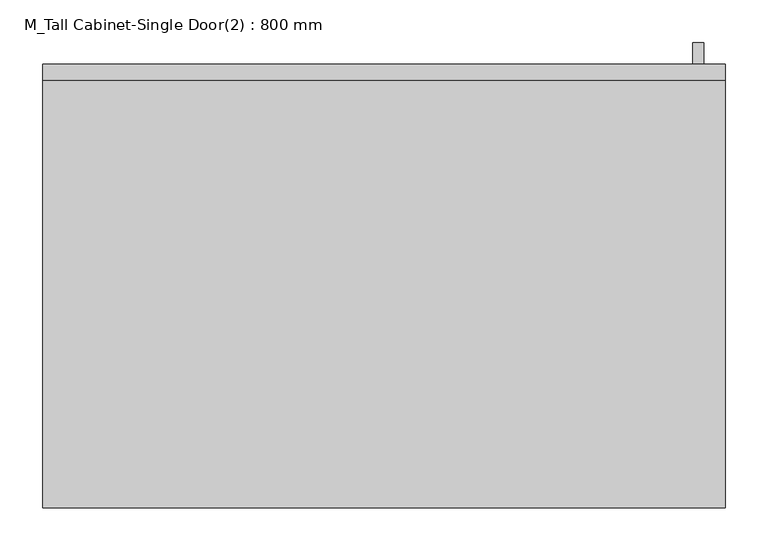
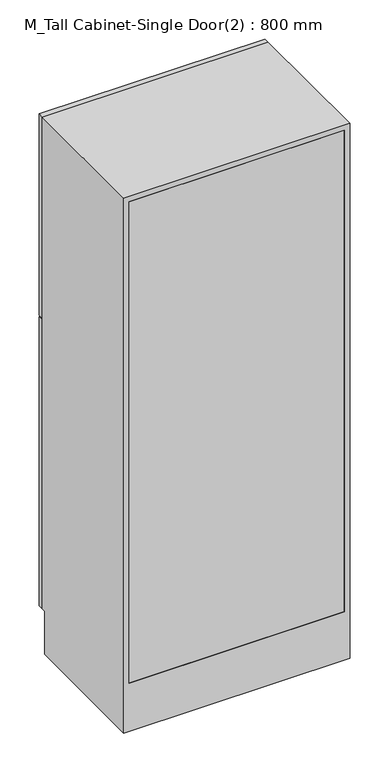
"""IFC4 building model written with IfcOpenShell, lengths in millimetres: furniture geometry, M_Tall Cabinet-Single Door(2) : 800 mm."""

from ifc_helpers import new_model, si_unit, frame, origin, place, context, project, spatial, polyline, outline, extrude, faceted_brep, source, transform, mapped, element, save


def m_tall_cabinet_single_door_2_800_mm_e6cfeb17(model_context):
    return source(origin(), model_context, "Body", "SolidModel", [
        faceted_brep([(418.7377049, 500.95, 161.5875), (-381.2622951, 500.95, 161.5875), (-381.2622951, 500.95, 2000.0), (418.7377049, 500.95, 2000.0), (399.6877049, 500.95, 1980.95), (-362.2122951, 500.95, 1980.95), (-362.2122951, 500.95, 180.6375), (399.6877049, 500.95, 180.6375), (-381.2622951, 0.0, 2000.0), (-381.2622951, 0.0, 0.0), (418.7377049, 0.0, 0.0), (418.7377049, 0.0, 2000.0), (399.6877049, 0.0, 1980.95), (399.6877049, 0.0, 180.6375), (-362.2122951, 0.0, 180.6375), (-362.2122951, 0.0, 1980.95), (418.7377049, 485.0, 0.0), (418.7377049, 485.0, 161.5875), (-381.2622951, 485.0, 161.5875), (-381.2622951, 485.0, 0.0)], [[[0, 1, 2, 3], [4, 5, 6, 7]], [[8, 9, 10, 11], [12, 13, 14, 15]], [[3, 11, 10, 16, 17, 0]], [[2, 8, 11, 3]], [[1, 18, 19, 9, 8, 2]], [[0, 17, 18, 1]], [[7, 13, 12, 4]], [[6, 14, 13, 7]], [[5, 15, 14, 6]], [[4, 12, 15, 5]], [[10, 9, 19, 16]], [[19, 18, 17, 16]]]),
        extrude(outline(polyline([(393.3377049, 545.4), (393.3377049, 520.0), (380.8054733, 520.0), (380.8054733, 545.4), (393.3377049, 545.4)])), frame((0.0, 0.0, 1269.9480367), z_axis=(0.0, 0.0, 1.0), x_axis=(1.0, 0.0, 0.0)), (0.0, 0.0, 1.0), 101.6),
        extrude(outline(polyline([(393.3377049, 545.4), (393.3377049, 520.0), (380.8054733, 520.0), (380.8054733, 545.4), (393.3377049, 545.4)])), frame((0.0, 0.0, 1117.5480367), z_axis=(0.0, 0.0, 1.0), x_axis=(1.0, 0.0, 0.0)), (0.0, 0.0, 1.0), 101.6),
        extrude(outline(polyline([(355.2377049, 507.3), (355.2377049, 500.95), (-317.7622951, 500.95), (-317.7622951, 507.3), (355.2377049, 507.3)])), frame((0.0, 0.0, 1308.0480367), z_axis=(0.0, 0.0, 1.0), x_axis=(1.0, 0.0, 0.0)), (0.0, 0.0, 1.0), 628.4519633),
        extrude(outline(polyline([(355.2377049, 507.3), (355.2377049, 500.95), (-317.7622951, 500.95), (-317.7622951, 507.3), (355.2377049, 507.3)])), frame((0.0, 0.0, 225.0875), z_axis=(0.0, 0.0, 1.0), x_axis=(1.0, 0.0, 0.0)), (0.0, 0.0, 1.0), 955.9605367),
        extrude(outline(polyline([(2000.0, 418.7377049), (2000.0, -381.2622951), (1247.7230367, -381.2622951), (1247.7230367, 418.7377049), (2000.0, 418.7377049)]), holes=[polyline([(1936.5, 355.2377049), (1308.0480367, 355.2377049), (1308.0480367, -317.7622951), (1936.5, -317.7622951), (1936.5, 355.2377049)])]), frame((0.0, 500.95, 0.0), z_axis=(0.0, 1.0, 0.0), x_axis=(0.0, 0.0, 1.0)), (0.0, 0.0, 1.0), 19.05),
        extrude(outline(polyline([(161.5875, 418.7377049), (1241.3730367, 418.7377049), (1241.3730367, -381.2622951), (161.5875, -381.2622951), (161.5875, 418.7377049)]), holes=[polyline([(1181.0480367, 355.2377049), (225.0875, 355.2377049), (225.0875, -317.7622951), (1181.0480367, -317.7622951), (1181.0480367, 355.2377049)])]), frame((0.0, 500.95, 0.0), z_axis=(0.0, 1.0, 0.0), x_axis=(0.0, 0.0, 1.0)), (0.0, 0.0, 1.0), 19.05),
        extrude(outline(polyline([(399.6877049, 19.05), (399.6877049, 0.0), (-362.2122951, 0.0), (-362.2122951, 19.05), (399.6877049, 19.05)])), frame((0.0, 0.0, 180.6375), z_axis=(0.0, 0.0, 1.0), x_axis=(1.0, 0.0, 0.0)), (0.0, 0.0, 1.0), 1800.3125),
    ])


if __name__ == "__main__":
    model = new_model("IFC4")
    model_context = context("Model", 3, world=origin())
    ifc_project = project(units=[si_unit("LENGTHUNIT", "METRE", prefix="MILLI")], contexts=[model_context])
    site = spatial("IfcSite", under=ifc_project)
    building = spatial("IfcBuilding", under=site)
    placement = place(None, origin())
    m_tall_cabinet_single_door_2_800_mm_shape = m_tall_cabinet_single_door_2_800_mm_e6cfeb17(model_context)
    element("IfcFurniture", 1, ObjectType="M_Tall Cabinet-Single Door(2) : 800 mm", at=placement, inside=building, context=model_context, shape_type="MappedRepresentation", body=[
        mapped(m_tall_cabinet_single_door_2_800_mm_shape, transform((0.0, 0.0, 0.0), x_axis=(1.0, 0.0, 0.0), y_axis=(0.0, 1.0, 0.0), z_axis=(0.0, 0.0, 1.0))),
    ])
    save(model, "model.ifc")

# Revit data of these elements
# Type "M_Tall Cabinet-Single Door(2) : 800 mm"
#   Manufacturer = "Manufacturer"
#   Finish = "Finish"
#   Construction Type = "Construction Type"
#   AccessibilityPerformance = "AccessibilityPerformance"
#   CodePerformance = "CodePerformance"
#   Area = "Area"
#   Color = "Color"
#   Constituents = "Constituents"
#   Features = "Features"
#   Finish = "Finish"
#   Grade = "Grade"
#   Material = "Material"
#   ModelReference = "ModelReference"
#   NominalHeight = "NominalHeight"
#   NominalLength = "NominalLength"
#   NominalWidth = "NominalWidth"
#   ProductionYear = "ProductionYear"
#   Reference = "Reference"
#   Shape = "Shape"
#   Size = "Size"
#   SustainabilityPerformance = "SustainabilityPerformance"
#   WarrantyDescription = "WarrantyDescription"
#   WarrantyDurationLabor = "WarrantyDurationLabor"
#   WarrantyDurationParts = "WarrantyDurationParts"
#   WarrantyGuarantorLabor = "WarrantyGuarantorLabor"
#   WarrantyGuarantorParts = "WarrantyGuarantorParts"
#   ExpectedLife = "ExpectedLife"
#   ReplacementCost = "ReplacementCost"
#   AssetAccountingType = "FIXED"
#   ModelLabel = "ModelLabel"
#   Depth = 0.520 m
#   Height = 2.000 m
#   Plinth Depth = 0.035 m
#   Plinth Height = 0.160 m
#   Width = 0.800 m
#   Cabinet Material = none
#   Door/Drawer Material = none
#   Handle Material = Cabinets - Handles
#   Panel Material = Cabinets - Panel
# Element 1 (IfcFurniture, "M_Tall Cabinet-Single Door(2) : 800 mm")
#   Materials on its faces: "Cabinets", "Cabinets - Handles", "Cabinets - Panel"
# Materials
#   "Cabinets - Handles": class "Metal", colour RGB 57 57 57, transparency 0
#   "Cabinets - Panel": class "Miscellaneous", colour RGB 249 249 249, transparency 0
#   "Cabinets": class "Miscellaneous", colour RGB 249 249 249, transparency 0
